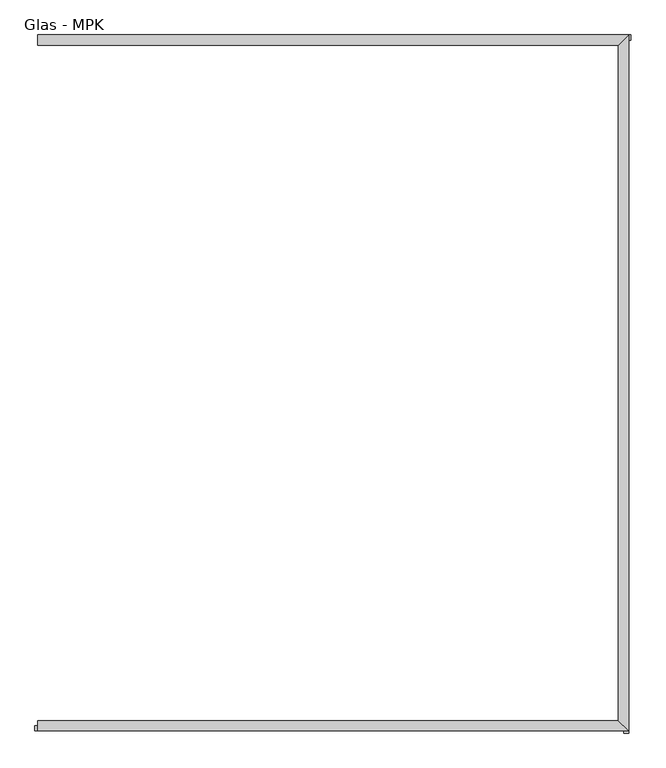
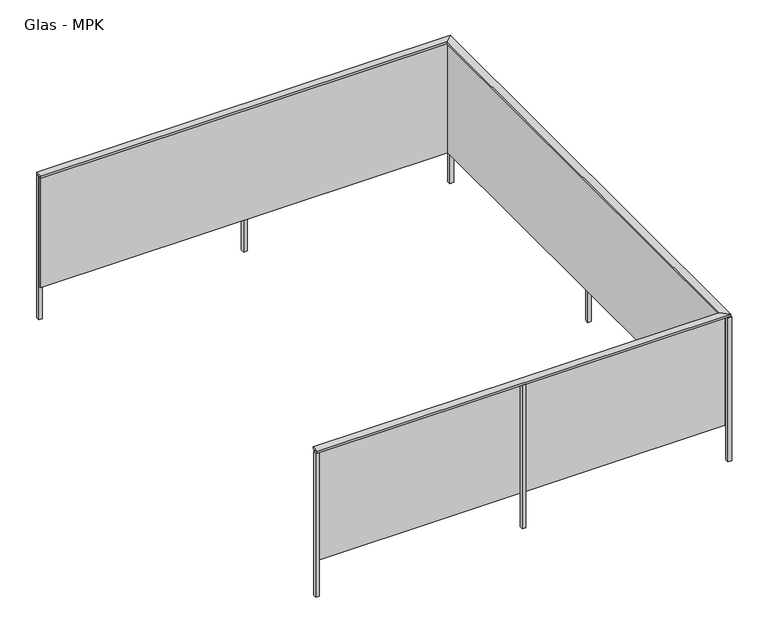
"""IFC4 building model written with IfcOpenShell, lengths in millimetres: railing geometry, Glas - MPK."""

from ifc_helpers import new_model, si_unit, frame, origin, place, context, project, spatial, polyline, outline, extrude, faceted_brep, source, transform, mapped, element, save


def glas_mpk_fba520f3(model_context):
    return source(origin(), model_context, "Body", "SolidModel", [
        faceted_brep([(29194.1667192, -1196.642277, 6843.2628643), (29194.1667192, -1246.642277, 6843.2628643), (29194.1667192, -1246.642277, 6856.7371357), (29194.1667192, -1196.642277, 6856.7371357), (32034.1667192, -1196.642277, 6843.2628643), (31984.1667192, -1246.642277, 6843.2628643), (31984.1667192, -1246.642277, 6856.7371357), (32034.1667192, -1196.642277, 6856.7371357), (32034.1667192, -4537.3716232, 6843.2628643), (31984.1667192, -4487.3716232, 6843.2628643), (31984.1667192, -4487.3716232, 6856.7371357), (32034.1667192, -4537.3716232, 6856.7371357), (29194.1667192, -4537.3716232, 6843.2628643), (29194.1667192, -4537.3716232, 6856.7371357), (29194.1667192, -4487.3716232, 6856.7371357), (29194.1667192, -4487.3716232, 6843.2628643)], [[[0, 1, 2, 3]], [[1, 0, 4, 5]], [[2, 1, 5, 6]], [[3, 2, 6, 7]], [[0, 3, 7, 4]], [[5, 4, 8, 9]], [[6, 5, 9, 10]], [[7, 6, 10, 11]], [[4, 7, 11, 8]], [[12, 13, 14, 15]], [[9, 8, 12, 15]], [[10, 9, 15, 14]], [[11, 10, 14, 13]], [[8, 11, 13, 12]]]),
        faceted_brep([(29194.1667192, -1236.642277, 6842.8769824), (29194.1667192, -1222.4501531, 6842.8769824), (29194.1667192, -1222.4501531, 6042.8769824), (29194.1667192, -1236.642277, 6042.8769824), (31994.1667192, -1236.642277, 6842.8769824), (32008.3588432, -1222.4501531, 6842.8769824), (32008.3588432, -1222.4501531, 6042.8769824), (31994.1667192, -1236.642277, 6042.8769824), (31994.1667192, -4497.3716232, 6842.8769824), (32008.3588432, -4511.5637472, 6842.8769824), (32008.3588432, -4511.5637472, 6042.8769824), (31994.1667192, -4497.3716232, 6042.8769824), (29194.1667192, -4497.3716232, 6842.8769824), (29194.1667192, -4497.3716232, 6042.8769824), (29194.1667192, -4511.5637472, 6042.8769824), (29194.1667192, -4511.5637472, 6842.8769824)], [[[0, 1, 2, 3]], [[1, 0, 4, 5]], [[2, 1, 5, 6]], [[3, 2, 6, 7]], [[0, 3, 7, 4]], [[5, 4, 8, 9]], [[6, 5, 9, 10]], [[7, 6, 10, 11]], [[4, 7, 11, 8]], [[12, 13, 14, 15]], [[9, 8, 12, 15]], [[10, 9, 15, 14]], [[11, 10, 14, 13]], [[8, 11, 13, 12]]]),
        extrude(outline(polyline([(30625.4167192, -4512.3716232), (30625.4167192, -4537.3716232), (30600.4167192, -4537.3716232), (30600.4167192, -4512.3716232), (30625.4167192, -4512.3716232)])), frame((0.0, 0.0, 5800.0), z_axis=(0.0, 0.0, 1.0), x_axis=(1.0, 0.0, 0.0)), (0.0, 0.0, 1.0), 1043.2628643),
        extrude(outline(polyline([(32009.1667192, -2854.5069501), (32034.1667192, -2854.5069501), (32034.1667192, -2879.5069501), (32009.1667192, -2879.5069501), (32009.1667192, -2854.5069501)])), frame((0.0, 0.0, 5800.0), z_axis=(0.0, 0.0, 1.0), x_axis=(1.0, 0.0, 0.0)), (0.0, 0.0, 1.0), 1043.2628643),
        extrude(outline(polyline([(30600.4167192, -1221.642277), (30600.4167192, -1196.642277), (30625.4167192, -1196.642277), (30625.4167192, -1221.642277), (30600.4167192, -1221.642277)])), frame((0.0, 0.0, 5800.0), z_axis=(0.0, 0.0, 1.0), x_axis=(1.0, 0.0, 0.0)), (0.0, 0.0, 1.0), 1043.2628643),
        extrude(outline(polyline([(32009.1667192, -4522.3716232), (32034.1667192, -4522.3716232), (32034.1667192, -4547.3716232), (32009.1667192, -4547.3716232), (32009.1667192, -4522.3716232)])), frame((0.0, 0.0, 5800.0), z_axis=(0.0, 0.0, 1.0), x_axis=(1.0, 0.0, 0.0)), (0.0, 0.0, 1.0), 1043.2628643),
        extrude(outline(polyline([(32019.1667192, -1221.642277), (32019.1667192, -1196.642277), (32044.1667192, -1196.642277), (32044.1667192, -1221.642277), (32019.1667192, -1221.642277)])), frame((0.0, 0.0, 5800.0), z_axis=(0.0, 0.0, 1.0), x_axis=(1.0, 0.0, 0.0)), (0.0, 0.0, 1.0), 1043.2628643),
        extrude(outline(polyline([(29206.6667192, -4512.3716232), (29206.6667192, -4537.3716232), (29181.6667192, -4537.3716232), (29181.6667192, -4512.3716232), (29206.6667192, -4512.3716232)])), frame((0.0, 0.0, 5800.0), z_axis=(0.0, 0.0, 1.0), x_axis=(1.0, 0.0, 0.0)), (0.0, 0.0, 1.0), 1043.2628643),
        extrude(outline(polyline([(29194.1667192, -1221.642277), (29194.1667192, -1196.642277), (29219.1667192, -1196.642277), (29219.1667192, -1221.642277), (29194.1667192, -1221.642277)])), frame((0.0, 0.0, 5800.0), z_axis=(0.0, 0.0, 1.0), x_axis=(1.0, 0.0, 0.0)), (0.0, 0.0, 1.0), 1043.2628643),
    ])


if __name__ == "__main__":
    model = new_model("IFC4")
    model_context = context("Model", 3, world=origin())
    ifc_project = project(units=[si_unit("LENGTHUNIT", "METRE", prefix="MILLI")], contexts=[model_context])
    site = spatial("IfcSite", under=ifc_project)
    building = spatial("IfcBuilding", under=site)
    placement = place(None, origin())
    glas_mpk_shape = glas_mpk_fba520f3(model_context)
    element("IfcRailing", 1, ObjectType="Glas - MPK", at=placement, inside=building, context=model_context, shape_type="MappedRepresentation", body=[
        mapped(glas_mpk_shape, transform((0.0, 0.0, 0.0), x_axis=(1.0, 0.0, 0.0), y_axis=(0.0, 1.0, 0.0), z_axis=(0.0, 0.0, 1.0))),
    ])
    save(model, "model.ifc")

# Revit data of these elements
# Element 1 (IfcRailing, "Glas - MPK")
#   Materials on its faces: "Metal - Aluminum", "Window - Glass"
# Materials
#   "Metal - Aluminum": class "Unassigned", colour RGB 247 247 247, transparency 0, Comments = "Rendering appearance not upgraded "
#   "Window - Glass": class "Glas", colour RGB 128 128 255, transparency 0.75
